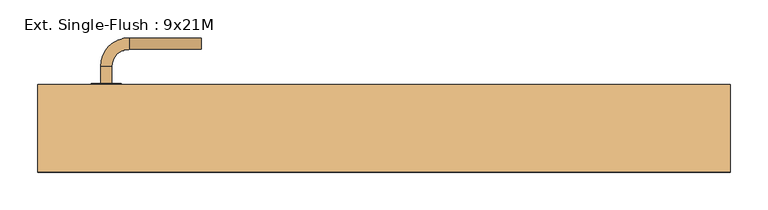
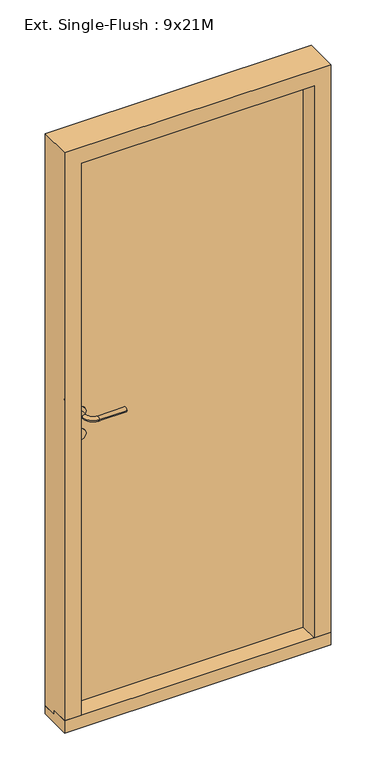
"""IFC4 building model written with IfcOpenShell, lengths in millimetres: door geometry, Ext. Single-Flush : 9x21M."""

import ifcopenshell
import ifcopenshell.guid

model = None  # the IFC model being written
_history = None  # IfcOwnerHistory: only IFC2X3 demands one
_inside = {}  # id of a spatial element -> (the spatial element, [elements in it])
_under = {}  # id of a project, library or spatial element -> (it, [spatial elements below it])
_declared = {}  # id of a project -> (the project, [libraries it declares])
_typed = {}  # id of a type object -> (the type object, [elements of that type])
_made_of = {}  # id of a material, layer set ... -> (it, [elements and type objects made of it])


def new_model(schema):
    """Start an empty IFC model of exactly this schema.

    Asked for "IFC4X3", IfcOpenShell would pick the latest addendum, in which some entities
    have other attributes; the version numbers below select the first issue.
    IFC2X3 requires an IfcOwnerHistory on every rooted entity: one is made here for all.
    """
    global model, _history
    if schema == "IFC4X3":
        model = ifcopenshell.file(schema_version=(4, 3, 0, 0))
    else:
        model = ifcopenshell.file(schema=schema)
    _inside.clear()
    _under.clear()
    _declared.clear()
    _typed.clear()
    _made_of.clear()
    _history = None
    if model.schema == "IFC2X3":
        org = make("IfcOrganization", Name="unknown")
        user = make(
            "IfcPersonAndOrganization",
            ThePerson=make("IfcPerson", FamilyName="unknown"),
            TheOrganization=org,
        )
        app = make(
            "IfcApplication",
            ApplicationDeveloper=org,
            Version="unknown",
            ApplicationFullName="unknown",
            ApplicationIdentifier="unknown",
        )
        _history = make(
            "IfcOwnerHistory",
            OwningUser=user,
            OwningApplication=app,
            ChangeAction="ADDED",
            CreationDate=0,
        )
    return model


def make(cls, **values):
    """One entity of the class cls with the attributes given. An attribute that is None is left unset."""
    return model.create_entity(
        cls, **{name: value for name, value in values.items() if value is not None}
    )


def rooted(cls, **values):
    """An entity with a GlobalId (a new one), such as an element, a storey or a relation."""
    return make(cls, GlobalId=ifcopenshell.guid.new(), OwnerHistory=_history, **values)


def si_unit(unit_type, name, prefix=None):
    """IfcSIUnit, for example si_unit("LENGTHUNIT", "METRE", prefix="MILLI")."""
    return make("IfcSIUnit", UnitType=unit_type, Prefix=prefix, Name=name)


def assignment(units):
    """IfcUnitAssignment: the units of a project."""
    return None if units is None else make("IfcUnitAssignment", Units=units)


def point(xyz):
    """IfcCartesianPoint."""
    return None if xyz is None else make("IfcCartesianPoint", Coordinates=xyz)


def direction(xyz):
    """IfcDirection."""
    return None if xyz is None else make("IfcDirection", DirectionRatios=xyz)


def frame(location, z_axis=None, x_axis=None):
    """IfcAxis2Placement3D, a coordinate frame: its origin and axes. An axis left out is left unset."""
    return make(
        "IfcAxis2Placement3D",
        Location=point(location),
        Axis=direction(z_axis),
        RefDirection=direction(x_axis),
    )


def frame_2d(location, x_axis=None):
    """IfcAxis2Placement2D, a coordinate frame in the plane: its origin and x axis."""
    return make(
        "IfcAxis2Placement2D", Location=point(location), RefDirection=direction(x_axis)
    )


def origin():
    """The frame at (0, 0, 0) with its axes left unset."""
    return frame((0.0, 0.0, 0.0))


def place(relative_to, where):
    """IfcLocalPlacement: puts the frame where relative to a parent placement (None: the world)."""
    return make(
        "IfcLocalPlacement", PlacementRelTo=relative_to, RelativePlacement=where
    )


def context(
    kind, dimensions, precision=None, world=None, true_north=None, identifier=None
):
    """IfcGeometricRepresentationContext, for example the 3D "Model" context."""
    return make(
        "IfcGeometricRepresentationContext",
        ContextIdentifier=identifier,
        ContextType=kind,
        CoordinateSpaceDimension=dimensions,
        Precision=precision,
        WorldCoordinateSystem=world,
        TrueNorth=true_north,
    )


def project(units=None, contexts=None):
    """IfcProject with its units and contexts."""
    return rooted(
        "IfcProject",
        Name="project",
        RepresentationContexts=contexts,
        UnitsInContext=assignment(units),
    )


def spatial(cls, under=None, at=None, **own):
    """A site, building, storey or space (cls), placed at a placement, below another one or the project."""
    s = rooted(cls, ObjectPlacement=at, **own)
    if under is not None:
        _under.setdefault(under.id(), (under, []))[1].append(s)
    return s


def polyline(points):
    """IfcPolyline through the points."""
    return make("IfcPolyline", Points=[point(p) for p in points])


def circle_curve(where, radius):
    """IfcCircle in the frame where."""
    return make("IfcCircle", Position=where, Radius=radius)


def ellipse_curve(where, semi_axis1, semi_axis2):
    """IfcEllipse in the frame where."""
    return make(
        "IfcEllipse", Position=where, SemiAxis1=semi_axis1, SemiAxis2=semi_axis2
    )


def trimmed(basis, trim1, trim2, sense, master):
    """IfcTrimmedCurve: the piece of a basis curve between two trims."""
    return make(
        "IfcTrimmedCurve",
        BasisCurve=basis,
        Trim1=trim1,
        Trim2=trim2,
        SenseAgreement=sense,
        MasterRepresentation=master,
    )


def segment(curve, same_sense, transition):
    """IfcCompositeCurveSegment."""
    return make(
        "IfcCompositeCurveSegment",
        Transition=transition,
        SameSense=same_sense,
        ParentCurve=curve,
    )


def composite_curve(segments, self_intersect=None):
    """IfcCompositeCurve: segments joined end to end."""
    return make("IfcCompositeCurve", Segments=segments, SelfIntersect=self_intersect)


def outline(outer, holes=None, kind="AREA"):
    """IfcArbitraryClosedProfileDef: a profile drawn as a closed curve; with holes, ...WithVoids."""
    if holes is None:
        return make("IfcArbitraryClosedProfileDef", ProfileType=kind, OuterCurve=outer)
    return make(
        "IfcArbitraryProfileDefWithVoids",
        ProfileType=kind,
        OuterCurve=outer,
        InnerCurves=holes,
    )


def extrude(swept, where, along, depth):
    """IfcExtrudedAreaSolid: the profile swept, set in the frame where, extruded along a direction by depth."""
    return make(
        "IfcExtrudedAreaSolid",
        SweptArea=swept,
        Position=where,
        ExtrudedDirection=direction(along),
        Depth=depth,
    )


def faces_of(points, faces, orient=None, outer=None):
    """IfcFace entities. A face is a list of loops; a loop is a list of indices into points, from 0.

    orient and outer hold one flag for each loop. By default every Orientation is true, the
    first loop of a face is its IfcFaceOuterBound and the others are IfcFaceBound.
    """
    made = []
    for i, loops in enumerate(faces):
        bounds = []
        for j, loop in enumerate(loops):
            is_outer = j == 0 if outer is None else outer[i][j]
            bounds.append(
                make(
                    "IfcFaceOuterBound" if is_outer else "IfcFaceBound",
                    Bound=make("IfcPolyLoop", Polygon=[points[k] for k in loop]),
                    Orientation=True if orient is None else orient[i][j],
                )
            )
        made.append(make("IfcFace", Bounds=bounds))
    return made


def faceted_brep(points, faces, orient=None, outer=None, voids=None):
    """IfcFacetedBrep: a solid bounded by flat faces; with voids (closed shells), ...WithVoids."""
    shared = [point(p) for p in points]
    hull = make("IfcClosedShell", CfsFaces=faces_of(shared, faces, orient, outer))
    if voids is None:
        return make("IfcFacetedBrep", Outer=hull)
    return make(
        "IfcFacetedBrepWithVoids",
        Outer=hull,
        Voids=[
            make(cls, CfsFaces=faces_of(shared, fs, o, b)) for cls, fs, o, b in voids
        ],
    )


def shape(context_of_items, identifier, shape_type, items):
    """IfcShapeRepresentation: the items that make up one representation, for example the "Body"."""
    return make(
        "IfcShapeRepresentation",
        ContextOfItems=context_of_items,
        RepresentationIdentifier=identifier,
        RepresentationType=shape_type,
        Items=items,
    )


def source(mapping_origin, context_of_items, identifier, shape_type, items):
    """IfcRepresentationMap: a shape defined once, which mapped items show again and again."""
    return make(
        "IfcRepresentationMap",
        MappingOrigin=mapping_origin,
        MappedRepresentation=shape(context_of_items, identifier, shape_type, items),
    )


def transform(
    local_origin,
    x_axis=None,
    y_axis=None,
    z_axis=None,
    scale=None,
    scale2=None,
    scale3=None,
    uniform=True,
):
    """IfcCartesianTransformationOperator3D, or its non-uniform kind. x_axis, y_axis, z_axis: its Axis1, 2, 3."""
    if uniform:
        return make(
            "IfcCartesianTransformationOperator3D",
            Axis1=direction(x_axis),
            Axis2=direction(y_axis),
            LocalOrigin=point(local_origin),
            Scale=scale,
            Axis3=direction(z_axis),
        )
    return make(
        "IfcCartesianTransformationOperator3DnonUniform",
        Axis1=direction(x_axis),
        Axis2=direction(y_axis),
        LocalOrigin=point(local_origin),
        Scale=scale,
        Axis3=direction(z_axis),
        Scale2=scale2,
        Scale3=scale3,
    )


def mapped(mapping_source, mapping_target):
    """IfcMappedItem: shows the shape of a source again, moved by a transform."""
    return make(
        "IfcMappedItem", MappingSource=mapping_source, MappingTarget=mapping_target
    )


def made_of(thing, what):
    """Note that an element or type object is made of a material, layer set ...; save() writes the relation."""
    if what is not None:
        _made_of.setdefault(what.id(), (what, []))[1].append(thing)
    return thing


def element(
    cls,
    number,
    at=None,
    inside=None,
    cuts=None,
    type_object=None,
    material=None,
    context=None,
    identifier="Body",
    shape_type=None,
    held_by="IfcProductDefinitionShape",
    body=None,
    shapes=None,
    **own,
):
    """One element of the class cls, such as IfcWall. Its Tag is "e" and its number.

    at: its placement. inside: the storey or other place that contains it. cuts: it is an
    opening in that element (IfcRelVoidsElement). A single representation is given by context,
    identifier, shape_type and body (its items); several are given by shapes. held_by: the class
    of the entity that holds the representations. save() writes the other relations.
    """
    e = rooted(cls, Tag="e%d" % number, ObjectPlacement=at, **own)
    if body is not None:
        shapes = [shape(context, identifier, shape_type, body)]
    if shapes is not None:
        e.Representation = make(held_by, Representations=shapes)
    if inside is not None:
        _inside.setdefault(inside.id(), (inside, []))[1].append(e)
    if cuts is not None:
        rooted(
            "IfcRelVoidsElement", RelatingBuildingElement=cuts, RelatedOpeningElement=e
        )
    if type_object is not None:
        _typed.setdefault(type_object.id(), (type_object, []))[1].append(e)
    return made_of(e, material)


def aggregate(whole, parts):
    """IfcRelAggregates: a whole, such as a stair, and the parts it consists of."""
    return rooted("IfcRelAggregates", RelatingObject=whole, RelatedObjects=parts)


def save(model, path):
    """Write the relations noted so far, then the file.

    IfcRelAggregates (storeys below a building ...), IfcRelContainedInSpatialStructure (elements
    in a storey), IfcRelDefinesByType, IfcRelAssociatesMaterial and IfcRelDeclares: one each for
    every whole, place, type object, material and project.
    """
    for whole, parts in _under.values():
        aggregate(whole, parts)
    for where, things in _inside.values():
        rooted(
            "IfcRelContainedInSpatialStructure",
            RelatedElements=things,
            RelatingStructure=where,
        )
    for kind, things in _typed.values():
        rooted("IfcRelDefinesByType", RelatedObjects=things, RelatingType=kind)
    for what, things in _made_of.values():
        rooted("IfcRelAssociatesMaterial", RelatedObjects=things, RelatingMaterial=what)
    for by, libraries in _declared.values():
        rooted("IfcRelDeclares", RelatingContext=by, RelatedDefinitions=libraries)
    model.write(path)


def plane_surface(at):
    """IfcPlane: the flat surface through the origin of the frame at, square to its z axis."""
    return make("IfcPlane", Position=at)


def cylinder_surface(at, radius):
    """IfcCylindricalSurface: all points at the distance radius from the z axis of the frame at."""
    return make("IfcCylindricalSurface", Position=at, Radius=radius)


def revolved_surface(curve, axis_point, axis_direction):
    """IfcSurfaceOfRevolution: the curve turned about the line through axis_point along axis_direction."""
    return make(
        "IfcSurfaceOfRevolution",
        SweptCurve=make("IfcArbitraryOpenProfileDef", ProfileType="CURVE", Curve=curve),
        AxisPosition=make("IfcAxis1Placement", Location=point(axis_point), Axis=direction(axis_direction)),
    )


def advanced_brep(points, edges, surfaces, faces):
    """IfcAdvancedBrep: a solid bounded by faces that lie on surfaces and meet in shared edges.

    An edge is (start, end): straight between two places in points (the first is 0);
    or (start, end, curve); or (start, end, curve, False) where it runs against its curve.
    A face is (place in surfaces, loops), or (place, loops, False) where it looks against
    its surface's normal. A loop lists edges by number (the first is 1), with a minus sign
    where the edge is run from its end to its start. The first loop is the outer one.
    """
    corners = [point(p) for p in points]
    vertices = [make("IfcVertexPoint", VertexGeometry=c) for c in corners]
    made = []
    for start, end, *more in edges:
        made.append(
            make(
                "IfcEdgeCurve",
                EdgeStart=vertices[start],
                EdgeEnd=vertices[end],
                EdgeGeometry=more[0] if more else make("IfcPolyline", Points=[corners[start], corners[end]]),
                SameSense=more[1] if len(more) > 1 else True,
            )
        )
    hull = []
    for where, loops, *sense in faces:
        bounds = []
        for j, loop in enumerate(loops):
            ring = [make("IfcOrientedEdge", EdgeElement=made[abs(k) - 1], Orientation=k > 0) for k in loop]
            bounds.append(
                make(
                    "IfcFaceOuterBound" if j == 0 else "IfcFaceBound",
                    Bound=make("IfcEdgeLoop", EdgeList=ring),
                    Orientation=True,
                )
            )
        hull.append(make("IfcAdvancedFace", Bounds=bounds, FaceSurface=surfaces[where], SameSense=sense[0] if sense else True))
    return make("IfcAdvancedBrep", Outer=make("IfcClosedShell", CfsFaces=hull))


def ext_single_flush_9x21m_44480e6f(model_context):
    return source(origin(), model_context, "Body", "SolidModel", [
        extrude(outline(composite_curve([segment(trimmed(circle_curve(frame_2d((1090.0, -366.0)), 20.0), [point((1070.0, -366.0))], [point((1110.0, -366.0))], False, "CARTESIAN"), True, "CONTINUOUS"), segment(trimmed(circle_curve(frame_2d((1090.0, -366.0)), 20.0), [point((1110.0, -366.0))], [point((1070.0, -366.0))], False, "CARTESIAN"), True, "CONTINUOUS")], self_intersect=False)), frame((0.0, 184.0, 0.0), z_axis=(0.0, 1.0, 0.0), x_axis=(0.0, 0.0, 1.0)), (0.0, 0.0, 1.0), 2.0),
        advanced_brep(
        [(-373.5, 186.0, 1090.0), (-358.5, 186.0, 1090.0), (-373.5, 208.5, 1090.0), (-358.5, 208.5, 1090.0), (-336.0, 231.0, 1090.0), (-336.0, 246.0, 1090.0), (-241.0, 246.0, 1090.0), (-241.0, 231.0, 1090.0)],
        [
            (0, 1, circle_curve(frame((-366.0, 186.0, 1090.0), z_axis=(0.0, -1.0, 0.0), x_axis=(1.0, 0.0, 0.0)), 7.5)),
            (1, 0, circle_curve(frame((-366.0, 186.0, 1090.0), z_axis=(0.0, -1.0, 0.0), x_axis=(1.0, 0.0, 0.0)), 7.5)),
            (0, 2),
            (2, 3, circle_curve(frame((-366.0, 208.5, 1090.0), z_axis=(0.0, -1.0, 0.0), x_axis=(1.0, 0.0, 0.0)), 7.5)),
            (3, 1),
            (3, 2, circle_curve(frame((-366.0, 208.5, 1090.0), z_axis=(0.0, -1.0, 0.0), x_axis=(1.0, 0.0, 0.0)), 7.5)),
            (4, 3, circle_curve(frame((-336.0, 208.5, 1090.0), z_axis=(0.0, 0.0, 1.0), x_axis=(-1.0, 0.0, 0.0)), 22.5)),
            (2, 5, circle_curve(frame((-336.0, 208.5, 1090.0), z_axis=(0.0, 0.0, -1.0), x_axis=(-1.0, 0.0, 0.0)), 37.5)),
            (5, 4, circle_curve(frame((-336.0, 238.5, 1090.0), z_axis=(-1.0, 0.0, 0.0), x_axis=(0.0, -1.0, 0.0)), 7.5)),
            (4, 5, circle_curve(frame((-336.0, 238.5, 1090.0), z_axis=(-1.0, 0.0, 0.0), x_axis=(0.0, -1.0, 0.0)), 7.5)),
            (5, 6),
            (6, 7, circle_curve(frame((-241.0, 238.5, 1090.0), z_axis=(-1.0, 0.0, 0.0), x_axis=(0.0, -1.0, 0.0)), 7.5)),
            (7, 4),
            (7, 6, circle_curve(frame((-241.0, 238.5, 1090.0), z_axis=(-1.0, 0.0, 0.0), x_axis=(0.0, -1.0, 0.0)), 7.5)),
        ],
        [
            plane_surface(frame((-366.0, 186.0, 1090.0), z_axis=(0.0, -1.0, 0.0), x_axis=(0.0, 0.0, -1.0))),
            cylinder_surface(frame((-366.0, 186.0, 1090.0), z_axis=(0.0, -1.0, 0.0), x_axis=(1.0, 0.0, 0.0)), 7.5),
            revolved_surface(trimmed(ellipse_curve(frame((-366.0, 208.5, 1090.0), z_axis=(0.0, -1.0, 0.0), x_axis=(1.0, 0.0, 0.0)), 7.5, 7.5), [point((-373.5, 208.5, 1090.0))], [point((-358.5, 208.5, 1090.0))], True, "CARTESIAN"), (-336.0, 208.5, 1090.0), (0.0, 0.0, -1.0)),
            revolved_surface(trimmed(ellipse_curve(frame((-366.0, 208.5, 1090.0), z_axis=(0.0, -1.0, 0.0), x_axis=(1.0, 0.0, 0.0)), 7.5, 7.5), [point((-358.5, 208.5, 1090.0))], [point((-373.5, 208.5, 1090.0))], True, "CARTESIAN"), (-336.0, 208.5, 1090.0), (0.0, 0.0, -1.0)),
            cylinder_surface(frame((-336.0, 238.5, 1090.0), z_axis=(-1.0, 0.0, 0.0), x_axis=(0.0, -1.0, 0.0)), 7.5),
            plane_surface(frame((-241.0, 238.5, 1090.0), z_axis=(1.0, 0.0, 0.0), x_axis=(0.0, 0.0, -1.0))),
        ],
        [
            (0, [[1, 2]]),
            (1, [[-1, 3, 4, 5]]),
            (1, [[-2, -5, 6, -3]]),
            (2, [[7, -4, 8, 9]]),
            (3, [[-8, -6, -7, 10]]),
            (4, [[-9, 11, 12, 13]]),
            (4, [[-10, -13, 14, -11]]),
            (5, [[-14, -12]]),
        ],
    ),
        extrude(outline(composite_curve([segment(trimmed(circle_curve(frame_2d((1010.0, -366.0)), 20.0), [point((990.0, -366.0))], [point((1030.0, -366.0))], False, "CARTESIAN"), True, "CONTINUOUS"), segment(trimmed(circle_curve(frame_2d((1010.0, -366.0)), 20.0), [point((1030.0, -366.0))], [point((990.0, -366.0))], False, "CARTESIAN"), True, "CONTINUOUS")], self_intersect=False), holes=[composite_curve([segment(trimmed(circle_curve(frame_2d((1015.0, -366.0)), 3.0), [point((1012.4019238, -367.5))], [point((1012.4019238, -364.5))], True, "CARTESIAN"), True, "CONTINUOUS"), segment(polyline([(1012.4019238, -364.5), (1000.0, -364.5), (1000.0, -367.5), (1012.4019238, -367.5)]), True, "CONTINUOUS")], self_intersect=False)]), frame((0.0, 184.0, 0.0), z_axis=(0.0, 1.0, 0.0), x_axis=(0.0, 0.0, 1.0)), (0.0, 0.0, 1.0), 2.0),
        extrude(outline(composite_curve([segment(trimmed(circle_curve(frame_2d((1090.0, -366.0)), 20.0), [point((1070.0, -366.0))], [point((1110.0, -366.0))], False, "CARTESIAN"), True, "CONTINUOUS"), segment(trimmed(circle_curve(frame_2d((1090.0, -366.0)), 20.0), [point((1110.0, -366.0))], [point((1070.0, -366.0))], False, "CARTESIAN"), True, "CONTINUOUS")], self_intersect=False)), frame((0.0, 132.0, 0.0), z_axis=(0.0, 1.0, 0.0), x_axis=(0.0, 0.0, 1.0)), (0.0, 0.0, 1.0), 2.0),
        advanced_brep(
        [(-373.5, 132.0, 1090.0), (-358.5, 132.0, 1090.0), (-358.5, 109.5, 1090.0), (-373.5, 109.5, 1090.0), (-336.0, 87.0, 1090.0), (-336.0, 72.0, 1090.0), (-241.0, 87.0, 1090.0), (-241.0, 72.0, 1090.0)],
        [
            (0, 1, circle_curve(frame((-366.0, 132.0, 1090.0), z_axis=(0.0, 1.0, 0.0), x_axis=(1.0, 0.0, 0.0)), 7.5)),
            (1, 0, circle_curve(frame((-366.0, 132.0, 1090.0), z_axis=(0.0, 1.0, 0.0), x_axis=(1.0, 0.0, 0.0)), 7.5)),
            (1, 2),
            (2, 3, circle_curve(frame((-366.0, 109.5, 1090.0), z_axis=(0.0, 1.0, 0.0), x_axis=(1.0, 0.0, 0.0)), 7.5)),
            (3, 0),
            (3, 2, circle_curve(frame((-366.0, 109.5, 1090.0), z_axis=(0.0, 1.0, 0.0), x_axis=(1.0, 0.0, 0.0)), 7.5)),
            (4, 5, circle_curve(frame((-336.0, 79.5, 1090.0), z_axis=(-1.0, 0.0, 0.0), x_axis=(0.0, 1.0, 0.0)), 7.5)),
            (5, 3, circle_curve(frame((-336.0, 109.5, 1090.0), z_axis=(0.0, 0.0, -1.0), x_axis=(-1.0, 0.0, 0.0)), 37.5)),
            (2, 4, circle_curve(frame((-336.0, 109.5, 1090.0), z_axis=(0.0, 0.0, 1.0), x_axis=(-1.0, 0.0, 0.0)), 22.5)),
            (5, 4, circle_curve(frame((-336.0, 79.5, 1090.0), z_axis=(-1.0, 0.0, 0.0), x_axis=(0.0, 1.0, 0.0)), 7.5)),
            (4, 6),
            (6, 7, circle_curve(frame((-241.0, 79.5, 1090.0), z_axis=(-1.0, 0.0, 0.0), x_axis=(0.0, 1.0, 0.0)), 7.5)),
            (7, 5),
            (7, 6, circle_curve(frame((-241.0, 79.5, 1090.0), z_axis=(-1.0, 0.0, 0.0), x_axis=(0.0, 1.0, 0.0)), 7.5)),
        ],
        [
            plane_surface(frame((-366.0, 132.0, 1090.0), z_axis=(0.0, 1.0, 0.0), x_axis=(0.0, 0.0, -1.0))),
            cylinder_surface(frame((-366.0, 132.0, 1090.0), z_axis=(0.0, 1.0, 0.0), x_axis=(1.0, 0.0, 0.0)), 7.5),
            revolved_surface(trimmed(ellipse_curve(frame((-366.0, 109.5, 1090.0), z_axis=(0.0, -1.0, 0.0), x_axis=(1.0, 0.0, 0.0)), 7.5, 7.5), [point((-373.5, 109.5, 1090.0))], [point((-358.5, 109.5, 1090.0))], True, "CARTESIAN"), (-336.0, 109.5, 1090.0), (0.0, 0.0, -1.0)),
            revolved_surface(trimmed(ellipse_curve(frame((-366.0, 109.5, 1090.0), z_axis=(0.0, -1.0, 0.0), x_axis=(1.0, 0.0, 0.0)), 7.5, 7.5), [point((-358.5, 109.5, 1090.0))], [point((-373.5, 109.5, 1090.0))], True, "CARTESIAN"), (-336.0, 109.5, 1090.0), (0.0, 0.0, -1.0)),
            cylinder_surface(frame((-336.0, 79.5, 1090.0), z_axis=(-1.0, 0.0, 0.0), x_axis=(0.0, 1.0, 0.0)), 7.5),
            plane_surface(frame((-241.0, 79.5, 1090.0), z_axis=(1.0, 0.0, 0.0), x_axis=(0.0, 0.0, -1.0))),
        ],
        [
            (0, [[1, 2]]),
            (1, [[3, 4, 5, -2]]),
            (1, [[-5, 6, -3, -1]]),
            (2, [[7, 8, -4, 9]]),
            (3, [[10, -9, -6, -8]]),
            (4, [[11, 12, 13, -7]]),
            (4, [[-13, 14, -11, -10]]),
            (5, [[-12, -14]]),
        ],
    ),
        extrude(outline(composite_curve([segment(trimmed(circle_curve(frame_2d((1010.0, -366.0)), 20.0), [point((990.0, -366.0))], [point((1030.0, -366.0))], False, "CARTESIAN"), True, "CONTINUOUS"), segment(trimmed(circle_curve(frame_2d((1010.0, -366.0)), 20.0), [point((1030.0, -366.0))], [point((990.0, -366.0))], False, "CARTESIAN"), True, "CONTINUOUS")], self_intersect=False), holes=[composite_curve([segment(trimmed(circle_curve(frame_2d((1015.0, -366.0)), 3.0), [point((1012.4019238, -367.5))], [point((1012.4019238, -364.5))], True, "CARTESIAN"), True, "CONTINUOUS"), segment(polyline([(1012.4019238, -364.5), (1000.0, -364.5), (1000.0, -367.5), (1012.4019238, -367.5)]), True, "CONTINUOUS")], self_intersect=False)]), frame((0.0, 132.0, 0.0), z_axis=(0.0, 1.0, 0.0), x_axis=(0.0, 0.0, 1.0)), (0.0, 0.0, 1.0), 2.0),
        extrude(outline(polyline([(-414.0, 184.0), (414.0, 184.0), (414.0, 134.0), (-414.0, 134.0), (-414.0, 184.0)])), frame((0.0, 0.0, 30.0), z_axis=(0.0, 0.0, 1.0), x_axis=(1.0, 0.0, 0.0)), (0.0, 0.0, 1.0), 2028.0),
        faceted_brep([(414.0, 184.0, 2058.0), (-414.0, 184.0, 2058.0), (-414.0, 184.0, 30.0), (-456.0, 184.0, 30.0), (-456.0, 184.0, 2100.0), (456.0, 184.0, 2100.0), (456.0, 184.0, 30.0), (414.0, 184.0, 30.0), (-414.0, 134.0, 2058.0), (-414.0, 134.0, 45.0), (-414.0, 134.0, 30.0), (456.0, 134.0, 30.0), (414.0, 134.0, 30.0), (-456.0, 134.0, 30.0), (-456.0, 69.0, 2100.0), (-456.0, 134.0, 45.0), (-456.0, 69.0, 45.0), (456.0, 69.0, 2100.0), (456.0, 69.0, 45.0), (456.0, 134.0, 45.0), (414.0, 134.0, 2058.0), (414.0, 134.0, 45.0), (-399.0, 69.0, 45.0), (-399.0, 69.0, 2043.0), (399.0, 69.0, 2043.0), (399.0, 69.0, 45.0), (399.0, 134.0, 45.0), (-399.0, 134.0, 45.0), (-399.0, 134.0, 2043.0), (399.0, 134.0, 2043.0)], [[[0, 1, 2, 3, 4, 5, 6, 7]], [[1, 8, 9, 10, 2]], [[11, 12, 7, 6]], [[10, 13, 3, 2]], [[14, 4, 3, 13, 15, 16]], [[5, 17, 18, 19, 11, 6]], [[20, 0, 7, 12, 21]], [[17, 14, 16, 22, 23, 24, 25, 18]], [[21, 19, 18, 25, 26]], [[15, 9, 27, 22, 16]], [[19, 21, 12, 11]], [[9, 15, 13, 10]], [[28, 23, 22, 27]], [[24, 29, 26, 25]], [[29, 28, 27, 9, 8, 20, 21, 26]], [[5, 4, 14, 17]], [[24, 23, 28, 29]], [[1, 0, 20, 8]]]),
        extrude(outline(polyline([(184.0, 30.0), (184.0, 0.0), (69.0, 0.0), (69.0, 45.0), (134.0, 45.0), (134.0, 30.0), (184.0, 30.0)])), frame((-456.0, 0.0, 0.0), z_axis=(1.0, 0.0, 0.0), x_axis=(0.0, 1.0, 0.0)), (0.0, 0.0, 1.0), 912.0),
    ])


if __name__ == "__main__":
    model = new_model("IFC4")
    model_context = context("Model", 3, world=origin())
    ifc_project = project(units=[si_unit("LENGTHUNIT", "METRE", prefix="MILLI")], contexts=[model_context])
    site = spatial("IfcSite", under=ifc_project)
    building = spatial("IfcBuilding", under=site)
    placement = place(None, origin())
    ext_single_flush_9x21m_shape = ext_single_flush_9x21m_44480e6f(model_context)
    element("IfcDoor", 1, ObjectType="Ext. Single-Flush : 9x21M", at=placement, inside=building, context=model_context, shape_type="MappedRepresentation", body=[
        mapped(ext_single_flush_9x21m_shape, transform((0.0, 0.0, 0.0), x_axis=(1.0, 0.0, 0.0), y_axis=(0.0, 1.0, 0.0), z_axis=(0.0, 0.0, 1.0))),
    ])
    save(model, "model.ifc")

# Revit data of these elements
# Project information
#   Client Name = "Test Project"
#   Project Address = "Enter address here"
#   Project Number = "Number"
#   Current Version = "0.0.0"
#   SR Document GUID = "3eb9317e-835d-4f79-8926-4d15b96bc824"
# Type "Ext. Single-Flush : 9x21M"
#   Type Mark = "51"
#   Sound Rating = ""
#   Opening Side [instance default] = ""
#   Hinge Side [instance default] = ""
#   Creator Organization [instance default] = "© Danish Educational Content"
#   Creator Name [instance default] = "© Erik Falck Jørgensen"
#   Creator Build [instance default] = "2017.0301.0"
#   Analytic Construction = "<None>"
#   length#6 = -50 mm
#   length#5 = 912 mm
#   length#4 = 120 mm
#   length#3 = 30 mm
#   length#2 = 57 mm
#   length#1 = 0 mm
#   Thickness = 50 mm
#   Seal Width = 12 mm
#   Rough Width = 912 mm
#   Rough Height = 2100 mm
#   Rebate Depth = 50 mm
#   Rabbet Width = 15 mm
#   Rabbet Depth = 50 mm
#   Height = 2088 mm
#   Width = 888 mm
#   Handle From Side = 90 mm
#   Handle From Bottom = 1090 mm
#   Exterior Direction [instance default] = 0.00°
#   Case Width = 45 mm
#   Case Depth = 115 mm
#   Threshold = yes
#   Sealing = no
#   Hinging = yes
#   Wall Closure = 1
#   Function = 1
#   Panel = none
#   Handle Finish = none
#   Handle = element 507533
#   Embrasure Interior = none
#   Embrasure Exterior = none
#   Case/Transom = none
#   Assembly Code = ""
# Element 1 (IfcDoor, "Ext. Single-Flush : 9x21M")
#   Materials on its faces: "Stainless Steel, Polished", "Default Frame/Mullion (Interior/Exterior)", "Default Door Panel (Exterior/Interior)"
# Materials
#   "Stainless Steel, Polished": class "Metal", colour RGB 180 180 180, transparency 0, Description = "Rustfri stål, poleret", Cost = 0
#   "Default Frame/Mullion (Interior/Exterior)": class "Generic", colour RGB 205 205 205, transparency 0, Description = "Udefineret karm/ramme materiale", Cost = 0
#   "Default Door Panel (Exterior/Interior)": class "Generic", colour RGB 205 205 205, transparency 0, Description = "Udefineret dørplade materiale", Cost = 0
